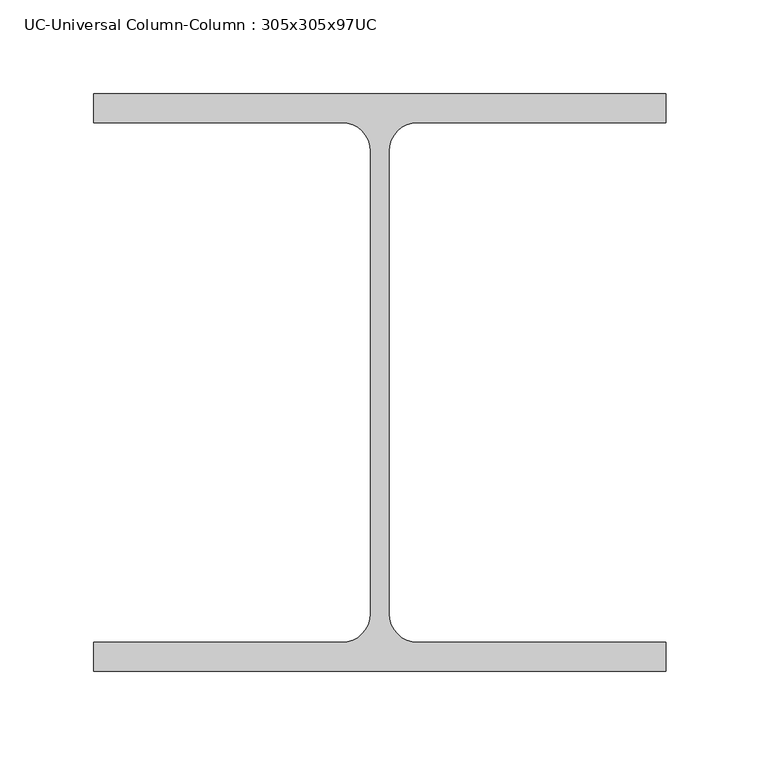
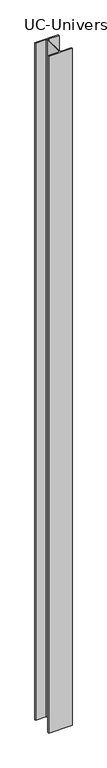
"""IFC4 building model written with IfcOpenShell, lengths in millimetres: column geometry, UC-Universal Column-Column : 305x305x97UC."""

from ifc_helpers import new_model, si_unit, point, frame, frame_2d, origin, place, context, project, spatial, polyline, circle_curve, trimmed, segment, composite_curve, outline, extrude, source, transform, mapped, element, save


def uc_universal_column_column_305x305x97uc_f4bfb62a(model_context):
    return source(origin(), model_context, "Body", "SweptSolid", [
        extrude(outline(composite_curve([segment(polyline([(152.65, 153.95), (152.65, 138.55), (20.15, 138.55)]), True, "CONTINUOUS"), segment(trimmed(circle_curve(frame_2d((20.15, 123.35)), 15.2), [point((20.15, 138.55))], [point((4.95, 123.35))], True, "CARTESIAN"), True, "CONTINUOUS"), segment(polyline([(4.95, 123.35), (4.95, -123.35)]), True, "CONTINUOUS"), segment(trimmed(circle_curve(frame_2d((20.15, -123.35)), 15.2), [point((4.95, -123.35))], [point((20.15, -138.55))], True, "CARTESIAN"), True, "CONTINUOUS"), segment(polyline([(20.15, -138.55), (152.65, -138.55), (152.65, -153.95), (-152.65, -153.95), (-152.65, -138.55), (-20.15, -138.55)]), True, "CONTINUOUS"), segment(trimmed(circle_curve(frame_2d((-20.15, -123.35)), 15.2), [point((-20.15, -138.55))], [point((-4.95, -123.35))], True, "CARTESIAN"), True, "CONTINUOUS"), segment(polyline([(-4.95, -123.35), (-4.95, 123.35)]), True, "CONTINUOUS"), segment(trimmed(circle_curve(frame_2d((-20.15, 123.35)), 15.2), [point((-4.95, 123.35))], [point((-20.15, 138.55))], True, "CARTESIAN"), True, "CONTINUOUS"), segment(polyline([(-20.15, 138.55), (-152.65, 138.55), (-152.65, 153.95), (152.65, 153.95)]), True, "CONTINUOUS")], self_intersect=False)), frame((0.0, 0.0, -1500.0), z_axis=(0.0, 0.0, 1.0), x_axis=(1.0, 0.0, 0.0)), (0.0, 0.0, 1.0), 9300.0),
    ])


if __name__ == "__main__":
    model = new_model("IFC4")
    model_context = context("Model", 3, world=origin())
    ifc_project = project(units=[si_unit("LENGTHUNIT", "METRE", prefix="MILLI")], contexts=[model_context])
    site = spatial("IfcSite", under=ifc_project)
    building = spatial("IfcBuilding", under=site)
    placement = place(None, origin())
    uc_universal_column_column_305x305x97uc_shape = uc_universal_column_column_305x305x97uc_f4bfb62a(model_context)
    element("IfcColumn", 1, ObjectType="UC-Universal Column-Column : 305x305x97UC", at=placement, inside=building, context=model_context, shape_type="MappedRepresentation", body=[
        mapped(uc_universal_column_column_305x305x97uc_shape, transform((0.0, 0.0, 0.0), x_axis=(1.0, 0.0, 0.0), y_axis=(0.0, 1.0, 0.0), z_axis=(0.0, 0.0, 1.0))),
    ])
    save(model, "model.ifc")

# Revit data of these elements
# Type "UC-Universal Column-Column : 305x305x97UC"
#   Keynote = "G10"
#   Nominal h = ""
#   W = 0
#   Ix = 0
#   M = 96.9
#   Zx = 0
#   b = 305.3 mm
#   h = 307.9 mm
#   r = 15.2 mm
#   s = 9.9 mm
#   t = 15.4 mm
#   A = 123 m²
#   Structural Material [instance default] = Steel, 45-345
#   Assembly Code = ""
# Element 1 (IfcColumn, "UC-Universal Column-Column : 305x305x97UC")
#   Materials on its faces: "Steel, 45-345"
# Materials
#   "Steel, 45-345": class "Metal", colour RGB 247 247 247, transparency 0, Description = "Steel 345 MPa", Cost = 0
